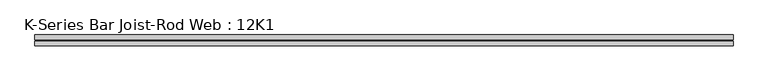
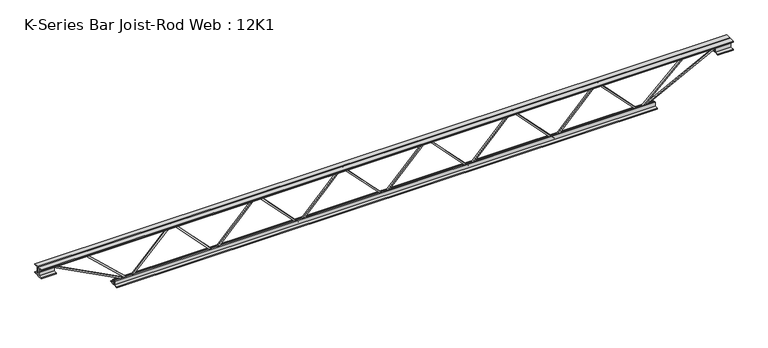
"""IFC4 building model written with IfcOpenShell, lengths in millimetres: beam geometry, K-Series Bar Joist-Rod Web : 12K1."""

import ifcopenshell
import ifcopenshell.guid

model = None  # the IFC model being written
_history = None  # IfcOwnerHistory: only IFC2X3 demands one
_inside = {}  # id of a spatial element -> (the spatial element, [elements in it])
_under = {}  # id of a project, library or spatial element -> (it, [spatial elements below it])
_declared = {}  # id of a project -> (the project, [libraries it declares])
_typed = {}  # id of a type object -> (the type object, [elements of that type])
_made_of = {}  # id of a material, layer set ... -> (it, [elements and type objects made of it])


def new_model(schema):
    """Start an empty IFC model of exactly this schema.

    Asked for "IFC4X3", IfcOpenShell would pick the latest addendum, in which some entities
    have other attributes; the version numbers below select the first issue.
    IFC2X3 requires an IfcOwnerHistory on every rooted entity: one is made here for all.
    """
    global model, _history
    if schema == "IFC4X3":
        model = ifcopenshell.file(schema_version=(4, 3, 0, 0))
    else:
        model = ifcopenshell.file(schema=schema)
    _inside.clear()
    _under.clear()
    _declared.clear()
    _typed.clear()
    _made_of.clear()
    _history = None
    if model.schema == "IFC2X3":
        org = make("IfcOrganization", Name="unknown")
        user = make(
            "IfcPersonAndOrganization",
            ThePerson=make("IfcPerson", FamilyName="unknown"),
            TheOrganization=org,
        )
        app = make(
            "IfcApplication",
            ApplicationDeveloper=org,
            Version="unknown",
            ApplicationFullName="unknown",
            ApplicationIdentifier="unknown",
        )
        _history = make(
            "IfcOwnerHistory",
            OwningUser=user,
            OwningApplication=app,
            ChangeAction="ADDED",
            CreationDate=0,
        )
    return model


def make(cls, **values):
    """One entity of the class cls with the attributes given. An attribute that is None is left unset."""
    return model.create_entity(
        cls, **{name: value for name, value in values.items() if value is not None}
    )


def rooted(cls, **values):
    """An entity with a GlobalId (a new one), such as an element, a storey or a relation."""
    return make(cls, GlobalId=ifcopenshell.guid.new(), OwnerHistory=_history, **values)


def si_unit(unit_type, name, prefix=None):
    """IfcSIUnit, for example si_unit("LENGTHUNIT", "METRE", prefix="MILLI")."""
    return make("IfcSIUnit", UnitType=unit_type, Prefix=prefix, Name=name)


def assignment(units):
    """IfcUnitAssignment: the units of a project."""
    return None if units is None else make("IfcUnitAssignment", Units=units)


def point(xyz):
    """IfcCartesianPoint."""
    return None if xyz is None else make("IfcCartesianPoint", Coordinates=xyz)


def direction(xyz):
    """IfcDirection."""
    return None if xyz is None else make("IfcDirection", DirectionRatios=xyz)


def frame(location, z_axis=None, x_axis=None):
    """IfcAxis2Placement3D, a coordinate frame: its origin and axes. An axis left out is left unset."""
    return make(
        "IfcAxis2Placement3D",
        Location=point(location),
        Axis=direction(z_axis),
        RefDirection=direction(x_axis),
    )


def origin():
    """The frame at (0, 0, 0) with its axes left unset."""
    return frame((0.0, 0.0, 0.0))


def place(relative_to, where):
    """IfcLocalPlacement: puts the frame where relative to a parent placement (None: the world)."""
    return make(
        "IfcLocalPlacement", PlacementRelTo=relative_to, RelativePlacement=where
    )


def context(
    kind, dimensions, precision=None, world=None, true_north=None, identifier=None
):
    """IfcGeometricRepresentationContext, for example the 3D "Model" context."""
    return make(
        "IfcGeometricRepresentationContext",
        ContextIdentifier=identifier,
        ContextType=kind,
        CoordinateSpaceDimension=dimensions,
        Precision=precision,
        WorldCoordinateSystem=world,
        TrueNorth=true_north,
    )


def project(units=None, contexts=None):
    """IfcProject with its units and contexts."""
    return rooted(
        "IfcProject",
        Name="project",
        RepresentationContexts=contexts,
        UnitsInContext=assignment(units),
    )


def spatial(cls, under=None, at=None, **own):
    """A site, building, storey or space (cls), placed at a placement, below another one or the project."""
    s = rooted(cls, ObjectPlacement=at, **own)
    if under is not None:
        _under.setdefault(under.id(), (under, []))[1].append(s)
    return s


def polyline(points):
    """IfcPolyline through the points."""
    return make("IfcPolyline", Points=[point(p) for p in points])


def outline(outer, holes=None, kind="AREA"):
    """IfcArbitraryClosedProfileDef: a profile drawn as a closed curve; with holes, ...WithVoids."""
    if holes is None:
        return make("IfcArbitraryClosedProfileDef", ProfileType=kind, OuterCurve=outer)
    return make(
        "IfcArbitraryProfileDefWithVoids",
        ProfileType=kind,
        OuterCurve=outer,
        InnerCurves=holes,
    )


def extrude(swept, where, along, depth):
    """IfcExtrudedAreaSolid: the profile swept, set in the frame where, extruded along a direction by depth."""
    return make(
        "IfcExtrudedAreaSolid",
        SweptArea=swept,
        Position=where,
        ExtrudedDirection=direction(along),
        Depth=depth,
    )


def shape(context_of_items, identifier, shape_type, items):
    """IfcShapeRepresentation: the items that make up one representation, for example the "Body"."""
    return make(
        "IfcShapeRepresentation",
        ContextOfItems=context_of_items,
        RepresentationIdentifier=identifier,
        RepresentationType=shape_type,
        Items=items,
    )


def source(mapping_origin, context_of_items, identifier, shape_type, items):
    """IfcRepresentationMap: a shape defined once, which mapped items show again and again."""
    return make(
        "IfcRepresentationMap",
        MappingOrigin=mapping_origin,
        MappedRepresentation=shape(context_of_items, identifier, shape_type, items),
    )


def transform(
    local_origin,
    x_axis=None,
    y_axis=None,
    z_axis=None,
    scale=None,
    scale2=None,
    scale3=None,
    uniform=True,
):
    """IfcCartesianTransformationOperator3D, or its non-uniform kind. x_axis, y_axis, z_axis: its Axis1, 2, 3."""
    if uniform:
        return make(
            "IfcCartesianTransformationOperator3D",
            Axis1=direction(x_axis),
            Axis2=direction(y_axis),
            LocalOrigin=point(local_origin),
            Scale=scale,
            Axis3=direction(z_axis),
        )
    return make(
        "IfcCartesianTransformationOperator3DnonUniform",
        Axis1=direction(x_axis),
        Axis2=direction(y_axis),
        LocalOrigin=point(local_origin),
        Scale=scale,
        Axis3=direction(z_axis),
        Scale2=scale2,
        Scale3=scale3,
    )


def mapped(mapping_source, mapping_target):
    """IfcMappedItem: shows the shape of a source again, moved by a transform."""
    return make(
        "IfcMappedItem", MappingSource=mapping_source, MappingTarget=mapping_target
    )


def made_of(thing, what):
    """Note that an element or type object is made of a material, layer set ...; save() writes the relation."""
    if what is not None:
        _made_of.setdefault(what.id(), (what, []))[1].append(thing)
    return thing


def element(
    cls,
    number,
    at=None,
    inside=None,
    cuts=None,
    type_object=None,
    material=None,
    context=None,
    identifier="Body",
    shape_type=None,
    held_by="IfcProductDefinitionShape",
    body=None,
    shapes=None,
    **own,
):
    """One element of the class cls, such as IfcWall. Its Tag is "e" and its number.

    at: its placement. inside: the storey or other place that contains it. cuts: it is an
    opening in that element (IfcRelVoidsElement). A single representation is given by context,
    identifier, shape_type and body (its items); several are given by shapes. held_by: the class
    of the entity that holds the representations. save() writes the other relations.
    """
    e = rooted(cls, Tag="e%d" % number, ObjectPlacement=at, **own)
    if body is not None:
        shapes = [shape(context, identifier, shape_type, body)]
    if shapes is not None:
        e.Representation = make(held_by, Representations=shapes)
    if inside is not None:
        _inside.setdefault(inside.id(), (inside, []))[1].append(e)
    if cuts is not None:
        rooted(
            "IfcRelVoidsElement", RelatingBuildingElement=cuts, RelatedOpeningElement=e
        )
    if type_object is not None:
        _typed.setdefault(type_object.id(), (type_object, []))[1].append(e)
    return made_of(e, material)


def aggregate(whole, parts):
    """IfcRelAggregates: a whole, such as a stair, and the parts it consists of."""
    return rooted("IfcRelAggregates", RelatingObject=whole, RelatedObjects=parts)


def save(model, path):
    """Write the relations noted so far, then the file.

    IfcRelAggregates (storeys below a building ...), IfcRelContainedInSpatialStructure (elements
    in a storey), IfcRelDefinesByType, IfcRelAssociatesMaterial and IfcRelDeclares: one each for
    every whole, place, type object, material and project.
    """
    for whole, parts in _under.values():
        aggregate(whole, parts)
    for where, things in _inside.values():
        rooted(
            "IfcRelContainedInSpatialStructure",
            RelatedElements=things,
            RelatingStructure=where,
        )
    for kind, things in _typed.values():
        rooted("IfcRelDefinesByType", RelatedObjects=things, RelatingType=kind)
    for what, things in _made_of.values():
        rooted("IfcRelAssociatesMaterial", RelatedObjects=things, RelatingMaterial=what)
    for by, libraries in _declared.values():
        rooted("IfcRelDeclares", RelatingContext=by, RelatedDefinitions=libraries)
    model.write(path)


def k_series_bar_joist_rod_web_12k1_bf9e2ae1(model_context):
    return source(origin(), model_context, "Body", "SweptSolid", [
        extrude(outline(polyline([(-141.2875, 571.5), (-150.8125, 571.5), (-150.8125, 576.7099667), (141.2875, 856.1099667), (141.2875, 858.3900333), (-150.8125, 1137.7900333), (-150.8125, 1143.0), (-141.2875, 1143.0), (-141.2875, 1141.8599667), (150.8125, 862.4599667), (150.8125, 852.0400333), (-141.2875, 572.6400333), (-141.2875, 571.5)])), frame((0.0, -4.7625, 0.0), z_axis=(0.0, 1.0, 0.0), x_axis=(0.0, 0.0, 1.0)), (0.0, 0.0, 1.0), 9.525),
        extrude(outline(polyline([(-141.2875, 0.0), (-150.8125, 0.0), (-150.8125, 5.2099667), (141.2875, 284.6099667), (141.2875, 286.8900333), (-150.8125, 566.2900333), (-150.8125, 571.5), (-141.2875, 571.5), (-141.2875, 570.3599667), (150.8125, 290.9599667), (150.8125, 280.5400333), (-141.2875, 1.1400333), (-141.2875, 0.0)])), frame((0.0, -4.7625, 0.0), z_axis=(0.0, 1.0, 0.0), x_axis=(0.0, 0.0, 1.0)), (0.0, 0.0, 1.0), 9.525),
        extrude(outline(polyline([(-141.2875, -571.5), (-150.8125, -571.5), (-150.8125, -566.2900333), (141.2875, -286.8900333), (141.2875, -284.6099667), (-150.8125, -5.2099667), (-150.8125, 0.0), (-141.2875, 0.0), (-141.2875, -1.1400333), (150.8125, -280.5400333), (150.8125, -290.9599667), (-141.2875, -570.3599667), (-141.2875, -571.5)])), frame((0.0, -4.7625, 0.0), z_axis=(0.0, 1.0, 0.0), x_axis=(0.0, 0.0, 1.0)), (0.0, 0.0, 1.0), 9.525),
        extrude(outline(polyline([(-141.2875, -1143.0), (-150.8125, -1143.0), (-150.8125, -1137.7900333), (141.2875, -858.3900333), (141.2875, -856.1099667), (-150.8125, -576.7099667), (-150.8125, -571.5), (-141.2875, -571.5), (-141.2875, -572.6400333), (150.8125, -852.0400333), (150.8125, -862.4599667), (-141.2875, -1141.8599667), (-141.2875, -1143.0)])), frame((0.0, -4.7625, 0.0), z_axis=(0.0, 1.0, 0.0), x_axis=(0.0, 0.0, 1.0)), (0.0, 0.0, 1.0), 9.525),
        extrude(outline(polyline([(-141.2875, 1143.0), (-150.8125, 1143.0), (-150.8125, 1148.2099667), (141.2875, 1427.6099667), (141.2875, 1429.8900333), (-150.8125, 1709.2900333), (-150.8125, 1714.5), (-141.2875, 1714.5), (-141.2875, 1713.3599667), (150.8125, 1433.9599667), (150.8125, 1423.5400333), (-141.2875, 1144.1400333), (-141.2875, 1143.0)])), frame((0.0, -4.7625, 0.0), z_axis=(0.0, 1.0, 0.0), x_axis=(0.0, 0.0, 1.0)), (0.0, 0.0, 1.0), 9.525),
        extrude(outline(polyline([(-141.2875, -1714.5), (-150.8125, -1714.5), (-150.8125, -1709.2900333), (141.2875, -1429.8900333), (141.2875, -1427.6099667), (-150.8125, -1148.2099667), (-150.8125, -1143.0), (-141.2875, -1143.0), (-141.2875, -1144.1400333), (150.8125, -1423.5400333), (150.8125, -1433.9599667), (-141.2875, -1713.3599667), (-141.2875, -1714.5)])), frame((0.0, -4.7625, 0.0), z_axis=(0.0, 1.0, 0.0), x_axis=(0.0, 0.0, 1.0)), (0.0, 0.0, 1.0), 9.525),
        extrude(outline(polyline([(4.7625, 152.4), (36.5125, 152.4), (36.5125, 146.05), (11.1125, 146.05), (11.1125, 120.65), (4.7625, 120.65), (4.7625, 152.4)])), frame((-2324.1, 0.0, 0.0), z_axis=(1.0, 0.0, 0.0), x_axis=(0.0, 1.0, 0.0)), (0.0, 0.0, 1.0), 4648.2),
        extrude(outline(polyline([(-4.7625, 152.4), (-4.7625, 120.65), (-11.1125, 120.65), (-11.1125, 146.05), (-36.5125, 146.05), (-36.5125, 152.4), (-4.7625, 152.4)])), frame((-2324.1, 0.0, 0.0), z_axis=(1.0, 0.0, 0.0), x_axis=(0.0, 1.0, 0.0)), (0.0, 0.0, 1.0), 4648.2),
        extrude(outline(polyline([(-4.7625, 88.9), (-36.5125, 88.9), (-36.5125, 95.25), (-11.1125, 95.25), (-11.1125, 120.65), (-4.7625, 120.65), (-4.7625, 88.9)])), frame((-2324.1, 0.0, 0.0), z_axis=(1.0, 0.0, 0.0), x_axis=(0.0, 1.0, 0.0)), (0.0, 0.0, 1.0), 101.6),
        extrude(outline(polyline([(36.5125, 88.9), (4.7625, 88.9), (4.7625, 120.65), (11.1125, 120.65), (11.1125, 95.25), (36.5125, 95.25), (36.5125, 88.9)])), frame((-2324.1, 0.0, 0.0), z_axis=(1.0, 0.0, 0.0), x_axis=(0.0, 1.0, 0.0)), (0.0, 0.0, 1.0), 101.6),
        extrude(outline(polyline([(4.7625, 88.9), (4.7625, 120.65), (11.1125, 120.65), (11.1125, 95.25), (36.5125, 95.25), (36.5125, 88.9), (4.7625, 88.9)])), frame((2222.5, 0.0, 0.0), z_axis=(1.0, 0.0, 0.0), x_axis=(0.0, 1.0, 0.0)), (0.0, 0.0, 1.0), 101.6),
        extrude(outline(polyline([(-4.7625, 88.9), (-36.5125, 88.9), (-36.5125, 95.25), (-11.1125, 95.25), (-11.1125, 120.65), (-4.7625, 120.65), (-4.7625, 88.9)])), frame((2222.5, 0.0, 0.0), z_axis=(1.0, 0.0, 0.0), x_axis=(0.0, 1.0, 0.0)), (0.0, 0.0, 1.0), 101.6),
        extrude(outline(polyline([(4.7625, -152.4), (4.7625, -120.65), (11.1125, -120.65), (11.1125, -146.05), (36.5125, -146.05), (36.5125, -152.4), (4.7625, -152.4)])), frame((-1816.1, 0.0, 0.0), z_axis=(1.0, 0.0, 0.0), x_axis=(0.0, 1.0, 0.0)), (0.0, 0.0, 1.0), 3632.2),
        extrude(outline(polyline([(-4.7625, -152.4), (-36.5125, -152.4), (-36.5125, -146.05), (-11.1125, -146.05), (-11.1125, -120.65), (-4.7625, -120.65), (-4.7625, -152.4)])), frame((-1816.1, 0.0, 0.0), z_axis=(1.0, 0.0, 0.0), x_axis=(0.0, 1.0, 0.0)), (0.0, 0.0, 1.0), 3632.2),
        extrude(outline(polyline([(0.0, -9.525), (0.0, 0.0), (573.7533355, 0.0), (573.7533355, -9.525), (0.0, -9.525)])), frame((-2224.7137714, 4.7625, 116.4332925), z_axis=(0.4648338989895134, 0.0, 0.8853979028381572), x_axis=(0.8853979028381572, 0.0, -0.4648338989895134)), (0.0, 0.0, 1.0), 9.525),
        extrude(outline(polyline([(0.0, -9.525), (0.0, 0.0), (390.8733203, 0.0), (390.8733203, -9.525), (0.0, -9.525)])), frame((-2003.4995407, 4.7625, 117.1683493), z_axis=(0.6823182503596337, 0.0, 0.7310552682432213), x_axis=(0.7310552682432213, 0.0, -0.6823182503596337)), (0.0, 0.0, 1.0), 9.525),
        extrude(outline(polyline([(0.0, -9.525), (0.0, 0.0), (573.7533355, 0.0), (573.7533355, -9.525), (0.0, -9.525)])), frame((2224.7137714, -4.7625, 116.4332925), z_axis=(-0.4648338989894951, 0.0, 0.8853979028381669), x_axis=(-0.8853979028381669, 0.0, -0.4648338989894951)), (0.0, 0.0, 1.0), 9.525),
        extrude(outline(polyline([(0.0, -9.525), (0.0, 0.0), (390.8733203, 0.0), (390.8733203, -9.525), (0.0, -9.525)])), frame((2003.4995407, -4.7625, 117.1683493), z_axis=(-0.6823182503596278, 0.0, 0.731055268243227), x_axis=(-0.731055268243227, 0.0, -0.6823182503596278)), (0.0, 0.0, 1.0), 9.525),
    ])


if __name__ == "__main__":
    model = new_model("IFC4")
    model_context = context("Model", 3, world=origin())
    ifc_project = project(units=[si_unit("LENGTHUNIT", "METRE", prefix="MILLI")], contexts=[model_context])
    site = spatial("IfcSite", under=ifc_project)
    building = spatial("IfcBuilding", under=site)
    placement = place(None, origin())
    k_series_bar_joist_rod_web_12k1_shape = k_series_bar_joist_rod_web_12k1_bf9e2ae1(model_context)
    element("IfcBeam", 1, ObjectType="K-Series Bar Joist-Rod Web : 12K1", at=placement, inside=building, context=model_context, shape_type="MappedRepresentation", body=[
        mapped(k_series_bar_joist_rod_web_12k1_shape, transform((0.0, 0.0, 0.0), x_axis=(1.0, 0.0, 0.0), y_axis=(0.0, 1.0, 0.0), z_axis=(0.0, 0.0, 1.0))),
    ])
    save(model, "model.ifc")

# Revit data of these elements
# Type "K-Series Bar Joist-Rod Web : 12K1"
#   Assembly Code = "B1010350"
#   Wt = 5
#   Web Thickness = 0' - 0 3/8"
#   Start Offset [instance default] = 0' - 0"
#   Start Extension [instance default] = 0' - 0"
#   Seat Length = 0' - 4"
#   Seat Depth = 0' - 2 1/2"
#   PanelArrayLength [instance default] = 20' - 0"
#   Panel [instance default] = 2' - 0"
#   End Offset [instance default] = 0' - 0"
#   End Extension [instance default] = 0' - 0"
#   End Panel = 2' - 0"
#   Cord Leg = 0' - 1 1/4"
#   Chord Thickness = 0' - 0 1/4"
#   Length [instance default] = 24' - 0"
#   Depth = 1' - 0"
#   PanelArrayNum [instance default] = 10
#   Structural Material = none
# Element 1 (IfcBeam, "K-Series Bar Joist-Rod Web : 12K1")
#   PanelArrayLength = 11' - 3"
#   Panel = 1' - 10 1/2"
#   PanelArrayNum = 6
